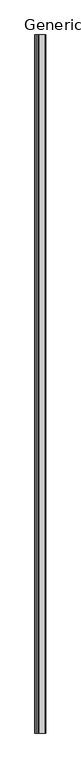
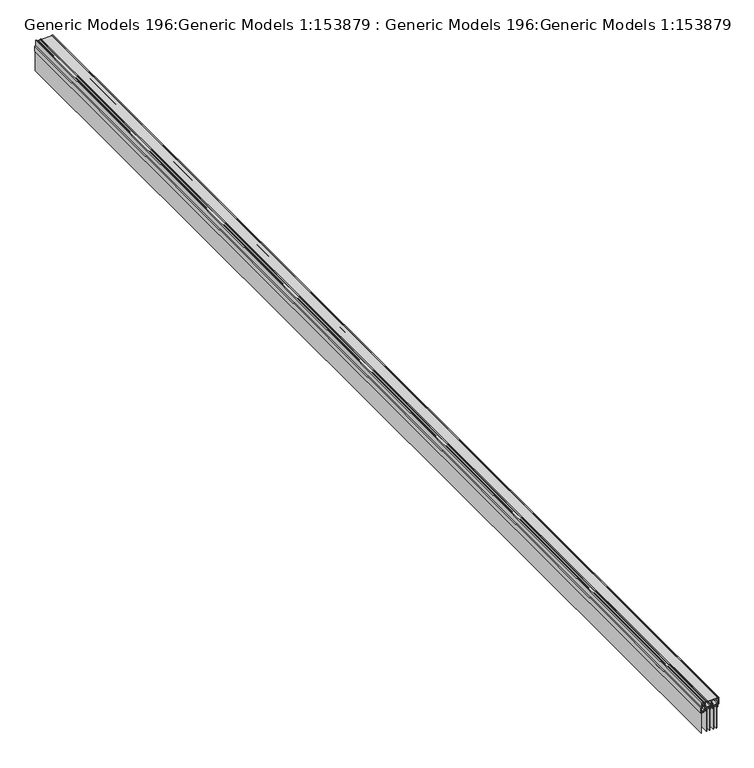
"""IFC4 building model written with IfcOpenShell, lengths in millimetres: proxy geometry, Generic Models 196:Generic Models 1:153879 : Generic Models 196:Generic Models 1:153879."""

from ifc_helpers import new_model, si_unit, frame, origin, place, context, project, spatial, polyline, outline, extrude, source, transform, mapped, element, save


def generic_models_196_generic_models_1_153879_generic_models_562f3e52(model_context):
    return source(origin(), model_context, "Body", "SweptSolid", [
        extrude(outline(polyline([(-5279.8266395, -273.9974793), (-5279.8266395, 7612.7025207), (-5265.496808, 7612.7025207), (-5265.496808, -273.9974793), (-5279.8266395, -273.9974793)])), frame((0.0, 0.0, 5862.6016649), z_axis=(0.0, 0.0, 1.0), x_axis=(1.0, 0.0, 0.0)), (0.0, 0.0, 1.0), 7.9798298),
        extrude(outline(polyline([(-5264.703058, -273.9974793), (-5264.703058, 7612.7025207), (-5259.9617238, 7612.7025207), (-5259.9617238, -273.9974793), (-5264.703058, -273.9974793)])), frame((0.0, 0.0, 5703.4496503), z_axis=(0.0, 0.0, 1.0), x_axis=(1.0, 0.0, 0.0)), (0.0, 0.0, 1.0), 167.9255943),
        extrude(outline(polyline([(-5285.3617238, -273.9974793), (-5285.3617238, 7612.7025207), (-5280.6203895, 7612.7025207), (-5280.6203895, -273.9974793), (-5285.3617238, -273.9974793)])), frame((0.0, 0.0, 5703.4496503), z_axis=(0.0, 0.0, 1.0), x_axis=(1.0, 0.0, 0.0)), (0.0, 0.0, 1.0), 167.9255943),
        extrude(outline(polyline([(5891.0179097, -5257.8450563), (5877.7252361, -5257.8450563), (5877.7252361, -5287.4783905), (5891.0179097, -5287.4783905), (5891.0179097, -5289.8490571), (5853.849243, -5289.8490571), (5853.849243, -5286.9703905), (5875.2699097, -5286.9703905), (5875.2699097, -5257.8450571), (5853.849243, -5257.8450571), (5853.849243, -5255.4743905), (5891.0179097, -5255.4743905), (5891.0179097, -5257.8450563)])), frame((0.0, -273.9974793, 0.0), z_axis=(0.0, 1.0, 0.0), x_axis=(0.0, 0.0, 1.0)), (0.0, 0.0, 1.0), 7886.7),
        extrude(outline(polyline([(-5328.1713019, -273.9974793), (-5328.1713019, 7612.7025207), (-5313.8414704, 7612.7025207), (-5313.8414704, -273.9974793), (-5328.1713019, -273.9974793)])), frame((0.0, 0.0, 5862.6016649), z_axis=(0.0, 0.0, 1.0), x_axis=(1.0, 0.0, 0.0)), (0.0, 0.0, 1.0), 7.9798298),
        extrude(outline(polyline([(-5313.0477204, -273.9974793), (-5313.0477204, 7612.7025207), (-5308.3063862, 7612.7025207), (-5308.3063862, -273.9974793), (-5313.0477204, -273.9974793)])), frame((0.0, 0.0, 5703.4496503), z_axis=(0.0, 0.0, 1.0), x_axis=(1.0, 0.0, 0.0)), (0.0, 0.0, 1.0), 167.9255943),
        extrude(outline(polyline([(-5333.7063862, -273.9974793), (-5333.7063862, 7612.7025207), (-5328.9650519, 7612.7025207), (-5328.9650519, -273.9974793), (-5333.7063862, -273.9974793)])), frame((0.0, 0.0, 5703.4496503), z_axis=(0.0, 0.0, 1.0), x_axis=(1.0, 0.0, 0.0)), (0.0, 0.0, 1.0), 167.9255943),
        extrude(outline(polyline([(5891.0179097, -5306.1897187), (5877.7252361, -5306.1897187), (5877.7252361, -5335.8230529), (5891.0179097, -5335.8230529), (5891.0179097, -5338.1937196), (5853.849243, -5338.1937196), (5853.849243, -5335.3150529), (5875.2699097, -5335.3150529), (5875.2699097, -5306.1897196), (5853.849243, -5306.1897196), (5853.849243, -5303.8190529), (5891.0179097, -5303.8190529), (5891.0179097, -5306.1897187)])), frame((0.0, -273.9974793, 0.0), z_axis=(0.0, 1.0, 0.0), x_axis=(0.0, 0.0, 1.0)), (0.0, 0.0, 1.0), 7886.7),
        extrude(outline(polyline([(5911.9895806, -5269.731065), (5912.7772369, -5268.9363724), (5913.7932292, -5268.3437221), (5913.7932292, -5253.0190554), (5913.6238958, -5252.0877221), (5913.0312292, -5251.3257221), (5912.2692292, -5250.7330554), (5911.3378958, -5250.5637221), (5884.2445667, -5250.3943716), (5884.2445667, -5252.0030399), (5873.4919087, -5252.0030399), (5873.4919087, -5247.8543716), (5921.2438975, -5247.8543716), (5921.2438975, -5254.2043732), (5919.6352309, -5254.2043732), (5919.6352309, -5249.6092823), (5918.1112309, -5249.8863732), (5917.2645642, -5250.4790399), (5916.7565642, -5251.2410399), (5916.5872447, -5252.1722972), (5916.5872447, -5331.6743913), (5919.6352361, -5331.6743913), (5919.6352361, -5327.187058), (5921.2439027, -5327.187058), (5921.2439027, -5333.537058), (5916.5025694, -5333.537058), (5915.6559027, -5360.207058), (5919.6352361, -5360.207058), (5919.6352361, -5355.8043913), (5921.2439027, -5355.8043913), (5921.2439027, -5362.1543913), (5887.8852309, -5362.1543913), (5887.8852309, -5360.2070563), (5913.793242, -5360.2070563), (5913.793242, -5345.3903766), (5913.6239087, -5344.4590433), (5913.031242, -5343.6970433), (5912.269242, -5343.1890433), (5911.3379087, -5342.9350433), (5873.4919087, -5342.9350433), (5873.4919087, -5339.1250477), (5883.2567859, -5339.1250477), (5884.244565, -5340.3950494), (5911.3379036, -5340.225716), (5912.2692369, -5340.0563827), (5913.0312369, -5339.463716), (5913.6239036, -5338.701716), (5913.7932369, -5337.7703827), (5913.7932369, -5325.3243827), (5912.7772369, -5324.731716), (5911.998378, -5323.902702), (5911.4332197, -5322.990427), (5911.0861774, -5322.0234162), (5910.9616661, -5321.0301952), (5911.0641012, -5320.0392893), (5911.3978979, -5319.0792238), (5911.96595, -5318.1770029), (5912.7772369, -5317.365716), (5913.7932438, -5316.6883879), (5913.7932438, -5297.8077152), (5884.2445667, -5297.8077152), (5884.2445667, -5299.670381), (5873.4919087, -5299.670381), (5873.4919087, -5293.3203732), (5884.244565, -5293.3203732), (5884.244565, -5295.1830391), (5913.7932369, -5294.9983599), (5913.7932369, -5276.8950391), (5912.7791924, -5276.300417), (5911.9864552, -5275.5076798), (5911.4225041, -5274.604938), (5911.0849371, -5273.6301634), (5910.9733078, -5272.6193724), (5911.0871695, -5271.6085814), (5911.426076, -5270.6338068), (5911.9895806, -5269.731065)])), frame((0.0, -273.9974793, 0.0), z_axis=(0.0, 1.0, 0.0), x_axis=(0.0, 0.0, 1.0)), (0.0, 0.0, 1.0), 7886.7),
        extrude(outline(polyline([(5845.0439113, -5368.6737177), (5845.0439113, -5367.0862177), (5703.4496503, -5367.0862177), (5703.4496503, -5366.2924677), (5845.0439113, -5366.2924677), (5845.0439113, -5347.9303785), (5851.2245753, -5347.9303785), (5851.2245753, -5344.8823732), (5904.0565686, -5344.8823732), (5904.0565686, -5346.1523776), (5891.1025789, -5346.1523776), (5891.1025789, -5357.3283776), (5904.0565789, -5357.3283776), (5904.0565789, -5358.5983913), (5883.9490282, -5358.5983913), (5881.3826715, -5368.6737177), (5845.0439113, -5368.6737177)]), holes=[polyline([(5889.832565, -5357.3283854), (5889.832565, -5346.2370382), (5862.2312464, -5346.2370382), (5862.2312464, -5356.3970494), (5860.6225694, -5356.3970494), (5860.6225694, -5346.1523862), (5852.4945667, -5346.1523862), (5852.4945667, -5349.2003913), (5846.3139044, -5349.2003913), (5846.3139044, -5360.1223879), (5852.494578, -5360.1223879), (5852.494578, -5367.319052), (5875.4392472, -5367.319052), (5875.4392472, -5364.9483854), (5876.7092283, -5364.9483854), (5876.7092283, -5367.319052), (5880.4562962, -5367.319052), (5882.9318596, -5357.3283854), (5889.832565, -5357.3283854)])]), frame((0.0, -273.9974793, 0.0), z_axis=(0.0, 1.0, 0.0), x_axis=(0.0, 0.0, 1.0)), (0.0, 0.0, 1.0), 7886.7),
    ])


if __name__ == "__main__":
    model = new_model("IFC4")
    model_context = context("Model", 3, world=origin())
    ifc_project = project(units=[si_unit("LENGTHUNIT", "METRE", prefix="MILLI")], contexts=[model_context])
    site = spatial("IfcSite", under=ifc_project)
    building = spatial("IfcBuilding", under=site)
    placement = place(None, origin())
    generic_models_196_generic_models_1_153879_generic_models_shape = generic_models_196_generic_models_1_153879_generic_models_562f3e52(model_context)
    element("IfcBuildingElementProxy", 1, Name="Generic Models 196:Generic Models 1:153879 : Generic Models 196:Generic Models 1:153879", ObjectType="Generic Models 196:Generic Models 1:153879 : Generic Models 196:Generic Models 1:153879", at=placement, inside=building, context=model_context, shape_type="MappedRepresentation", body=[
        mapped(generic_models_196_generic_models_1_153879_generic_models_shape, transform((0.0, 0.0, 0.0), x_axis=(1.0, 0.0, 0.0), y_axis=(0.0, 1.0, 0.0), z_axis=(0.0, 0.0, 1.0))),
    ])
    save(model, "model.ifc")

# Revit data of these elements
# Type "Generic Models 196:Generic Models 1:153879 : Generic Models 196:Generic Models 1:153879"
#   NameOverride = "Generic Models 196:Generic Models 1:153879"
#   ObjectTypeOverride = "Generic Models 196:Generic Models 1"
#   Reference = "Generic Models 1"
#   Category = "Generic Models"
#   Tag = "153879"
# Element 1 (IfcBuildingElementProxy, "Generic Models 196:Generic Models 1:153879 : Generic Models 196:Generic Models 1:153879")
#   Materials on its faces: "_SIDING DOOR PER SCHEDULE 11160"
# Materials
#   "_SIDING DOOR PER SCHEDULE 11160": class "Unassigned", colour RGB 255 255 255, transparency 0
